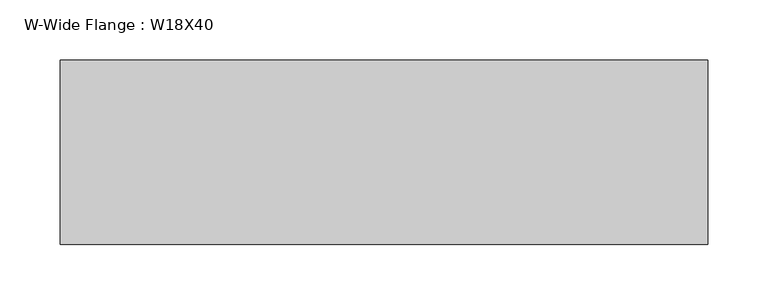
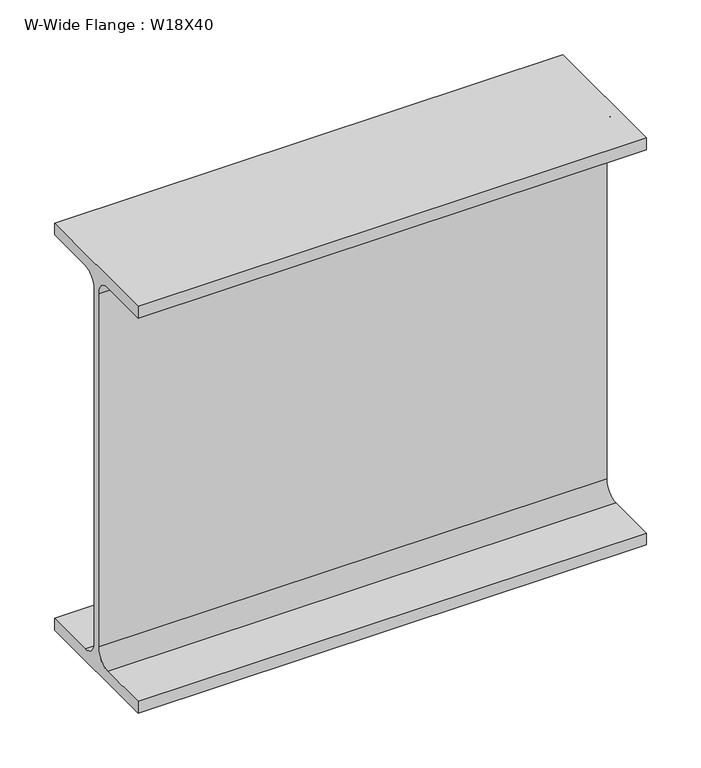
"""IFC4 building model written with IfcOpenShell, lengths in millimetres: beam geometry, W-Wide Flange : W18X40."""

from ifc_helpers import new_model, si_unit, point, frame, frame_2d, origin, place, context, project, spatial, polyline, circle_curve, trimmed, segment, composite_curve, outline, extrude, source, transform, mapped, element, save


def w_wide_flange_w18x40_b548adba(model_context):
    return source(origin(), model_context, "Body", "SweptSolid", [
        extrude(outline(composite_curve([segment(polyline([(76.454, -213.995), (76.454, -227.33), (-76.454, -227.33), (-76.454, -213.995), (-20.828, -213.995)]), True, "CONTINUOUS"), segment(trimmed(circle_curve(frame_2d((-20.828, -197.1675)), 16.8275), [point((-20.828, -213.995))], [point((-4.0005, -197.1675))], True, "CARTESIAN"), True, "CONTINUOUS"), segment(polyline([(-4.0005, -197.1675), (-4.0005, 197.1675)]), True, "CONTINUOUS"), segment(trimmed(circle_curve(frame_2d((-20.828, 197.1675)), 16.8275), [point((-4.0005, 197.1675))], [point((-20.828, 213.995))], True, "CARTESIAN"), True, "CONTINUOUS"), segment(polyline([(-20.828, 213.995), (-76.454, 213.995), (-76.454, 227.33), (76.454, 227.33), (76.454, 213.995), (20.828, 213.995)]), True, "CONTINUOUS"), segment(trimmed(circle_curve(frame_2d((20.828, 197.1675)), 16.8275), [point((20.828, 213.995))], [point((4.0005, 197.1675))], True, "CARTESIAN"), True, "CONTINUOUS"), segment(polyline([(4.0005, 197.1675), (4.0005, -197.1675)]), True, "CONTINUOUS"), segment(trimmed(circle_curve(frame_2d((20.828, -197.1675)), 16.8275), [point((4.0005, -197.1675))], [point((20.828, -213.995))], True, "CARTESIAN"), True, "CONTINUOUS"), segment(polyline([(20.828, -213.995), (76.454, -213.995)]), True, "CONTINUOUS")], self_intersect=False)), frame((-296.8625, 0.0, 0.0), z_axis=(1.0, 0.0, 0.0), x_axis=(0.0, 1.0, 0.0)), (0.0, 0.0, 1.0), 536.8925),
    ])


if __name__ == "__main__":
    model = new_model("IFC4")
    model_context = context("Model", 3, world=origin())
    ifc_project = project(units=[si_unit("LENGTHUNIT", "METRE", prefix="MILLI")], contexts=[model_context])
    site = spatial("IfcSite", under=ifc_project)
    building = spatial("IfcBuilding", under=site)
    placement = place(None, origin())
    w_wide_flange_w18x40_shape = w_wide_flange_w18x40_b548adba(model_context)
    element("IfcBeam", 1, ObjectType="W-Wide Flange : W18X40", at=placement, inside=building, context=model_context, shape_type="MappedRepresentation", body=[
        mapped(w_wide_flange_w18x40_shape, transform((0.0, 0.0, 0.0), x_axis=(1.0, 0.0, 0.0), y_axis=(0.0, 1.0, 0.0), z_axis=(0.0, 0.0, 1.0))),
    ])
    save(model, "model.ifc")

# Revit data of these elements
# Type "W-Wide Flange : W18X40"
#   Assembly Code = "B10"
#   W = 40
#   Length [instance default] = 5' - 0"
#   bf = 0' - 6.02"
#   d = 1' - 5.9"
#   k = 0' - 1 3/16"
#   k2 = 0' - 0.6625"
#   tf = 0' - 0.525"
#   tw = 0' - 0.315"
#   A = 0.0819444 SF
#   Structural Material [instance default] = Steel ASTM A992
# Element 1 (IfcBeam, "W-Wide Flange : W18X40")
#   Materials on its faces: "Steel ASTM A992"
# Materials
#   "Steel ASTM A992": class "Metal", colour RGB 199 199 199, transparency 0, Description = "Structural steel 50ksi", Cost = 0
